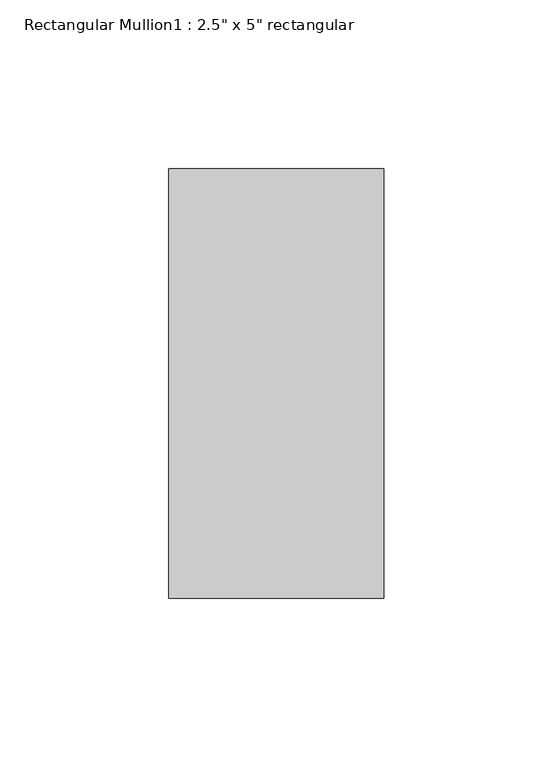
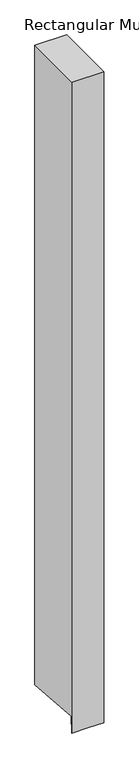
"""IFC4 building model written with IfcOpenShell, lengths in millimetres: member geometry."""

import ifcopenshell
import ifcopenshell.guid

model = None  # the IFC model being written
_history = None  # IfcOwnerHistory: only IFC2X3 demands one
_inside = {}  # id of a spatial element -> (the spatial element, [elements in it])
_under = {}  # id of a project, library or spatial element -> (it, [spatial elements below it])
_declared = {}  # id of a project -> (the project, [libraries it declares])
_typed = {}  # id of a type object -> (the type object, [elements of that type])
_made_of = {}  # id of a material, layer set ... -> (it, [elements and type objects made of it])


def new_model(schema):
    """Start an empty IFC model of exactly this schema.

    Asked for "IFC4X3", IfcOpenShell would pick the latest addendum, in which some entities
    have other attributes; the version numbers below select the first issue.
    IFC2X3 requires an IfcOwnerHistory on every rooted entity: one is made here for all.
    """
    global model, _history
    if schema == "IFC4X3":
        model = ifcopenshell.file(schema_version=(4, 3, 0, 0))
    else:
        model = ifcopenshell.file(schema=schema)
    _inside.clear()
    _under.clear()
    _declared.clear()
    _typed.clear()
    _made_of.clear()
    _history = None
    if model.schema == "IFC2X3":
        org = make("IfcOrganization", Name="unknown")
        user = make(
            "IfcPersonAndOrganization",
            ThePerson=make("IfcPerson", FamilyName="unknown"),
            TheOrganization=org,
        )
        app = make(
            "IfcApplication",
            ApplicationDeveloper=org,
            Version="unknown",
            ApplicationFullName="unknown",
            ApplicationIdentifier="unknown",
        )
        _history = make(
            "IfcOwnerHistory",
            OwningUser=user,
            OwningApplication=app,
            ChangeAction="ADDED",
            CreationDate=0,
        )
    return model


def make(cls, **values):
    """One entity of the class cls with the attributes given. An attribute that is None is left unset."""
    return model.create_entity(
        cls, **{name: value for name, value in values.items() if value is not None}
    )


def rooted(cls, **values):
    """An entity with a GlobalId (a new one), such as an element, a storey or a relation."""
    return make(cls, GlobalId=ifcopenshell.guid.new(), OwnerHistory=_history, **values)


def si_unit(unit_type, name, prefix=None):
    """IfcSIUnit, for example si_unit("LENGTHUNIT", "METRE", prefix="MILLI")."""
    return make("IfcSIUnit", UnitType=unit_type, Prefix=prefix, Name=name)


def assignment(units):
    """IfcUnitAssignment: the units of a project."""
    return None if units is None else make("IfcUnitAssignment", Units=units)


def point(xyz):
    """IfcCartesianPoint."""
    return None if xyz is None else make("IfcCartesianPoint", Coordinates=xyz)


def direction(xyz):
    """IfcDirection."""
    return None if xyz is None else make("IfcDirection", DirectionRatios=xyz)


def frame(location, z_axis=None, x_axis=None):
    """IfcAxis2Placement3D, a coordinate frame: its origin and axes. An axis left out is left unset."""
    return make(
        "IfcAxis2Placement3D",
        Location=point(location),
        Axis=direction(z_axis),
        RefDirection=direction(x_axis),
    )


def origin():
    """The frame at (0, 0, 0) with its axes left unset."""
    return frame((0.0, 0.0, 0.0))


def place(relative_to, where):
    """IfcLocalPlacement: puts the frame where relative to a parent placement (None: the world)."""
    return make(
        "IfcLocalPlacement", PlacementRelTo=relative_to, RelativePlacement=where
    )


def context(
    kind, dimensions, precision=None, world=None, true_north=None, identifier=None
):
    """IfcGeometricRepresentationContext, for example the 3D "Model" context."""
    return make(
        "IfcGeometricRepresentationContext",
        ContextIdentifier=identifier,
        ContextType=kind,
        CoordinateSpaceDimension=dimensions,
        Precision=precision,
        WorldCoordinateSystem=world,
        TrueNorth=true_north,
    )


def project(units=None, contexts=None):
    """IfcProject with its units and contexts."""
    return rooted(
        "IfcProject",
        Name="project",
        RepresentationContexts=contexts,
        UnitsInContext=assignment(units),
    )


def spatial(cls, under=None, at=None, **own):
    """A site, building, storey or space (cls), placed at a placement, below another one or the project."""
    s = rooted(cls, ObjectPlacement=at, **own)
    if under is not None:
        _under.setdefault(under.id(), (under, []))[1].append(s)
    return s


def faces_of(points, faces, orient=None, outer=None):
    """IfcFace entities. A face is a list of loops; a loop is a list of indices into points, from 0.

    orient and outer hold one flag for each loop. By default every Orientation is true, the
    first loop of a face is its IfcFaceOuterBound and the others are IfcFaceBound.
    """
    made = []
    for i, loops in enumerate(faces):
        bounds = []
        for j, loop in enumerate(loops):
            is_outer = j == 0 if outer is None else outer[i][j]
            bounds.append(
                make(
                    "IfcFaceOuterBound" if is_outer else "IfcFaceBound",
                    Bound=make("IfcPolyLoop", Polygon=[points[k] for k in loop]),
                    Orientation=True if orient is None else orient[i][j],
                )
            )
        made.append(make("IfcFace", Bounds=bounds))
    return made


def faceted_brep(points, faces, orient=None, outer=None, voids=None):
    """IfcFacetedBrep: a solid bounded by flat faces; with voids (closed shells), ...WithVoids."""
    shared = [point(p) for p in points]
    hull = make("IfcClosedShell", CfsFaces=faces_of(shared, faces, orient, outer))
    if voids is None:
        return make("IfcFacetedBrep", Outer=hull)
    return make(
        "IfcFacetedBrepWithVoids",
        Outer=hull,
        Voids=[
            make(cls, CfsFaces=faces_of(shared, fs, o, b)) for cls, fs, o, b in voids
        ],
    )


def shape(context_of_items, identifier, shape_type, items):
    """IfcShapeRepresentation: the items that make up one representation, for example the "Body"."""
    return make(
        "IfcShapeRepresentation",
        ContextOfItems=context_of_items,
        RepresentationIdentifier=identifier,
        RepresentationType=shape_type,
        Items=items,
    )


def source(mapping_origin, context_of_items, identifier, shape_type, items):
    """IfcRepresentationMap: a shape defined once, which mapped items show again and again."""
    return make(
        "IfcRepresentationMap",
        MappingOrigin=mapping_origin,
        MappedRepresentation=shape(context_of_items, identifier, shape_type, items),
    )


def transform(
    local_origin,
    x_axis=None,
    y_axis=None,
    z_axis=None,
    scale=None,
    scale2=None,
    scale3=None,
    uniform=True,
):
    """IfcCartesianTransformationOperator3D, or its non-uniform kind. x_axis, y_axis, z_axis: its Axis1, 2, 3."""
    if uniform:
        return make(
            "IfcCartesianTransformationOperator3D",
            Axis1=direction(x_axis),
            Axis2=direction(y_axis),
            LocalOrigin=point(local_origin),
            Scale=scale,
            Axis3=direction(z_axis),
        )
    return make(
        "IfcCartesianTransformationOperator3DnonUniform",
        Axis1=direction(x_axis),
        Axis2=direction(y_axis),
        LocalOrigin=point(local_origin),
        Scale=scale,
        Axis3=direction(z_axis),
        Scale2=scale2,
        Scale3=scale3,
    )


def mapped(mapping_source, mapping_target):
    """IfcMappedItem: shows the shape of a source again, moved by a transform."""
    return make(
        "IfcMappedItem", MappingSource=mapping_source, MappingTarget=mapping_target
    )


def made_of(thing, what):
    """Note that an element or type object is made of a material, layer set ...; save() writes the relation."""
    if what is not None:
        _made_of.setdefault(what.id(), (what, []))[1].append(thing)
    return thing


def element(
    cls,
    number,
    at=None,
    inside=None,
    cuts=None,
    type_object=None,
    material=None,
    context=None,
    identifier="Body",
    shape_type=None,
    held_by="IfcProductDefinitionShape",
    body=None,
    shapes=None,
    **own,
):
    """One element of the class cls, such as IfcWall. Its Tag is "e" and its number.

    at: its placement. inside: the storey or other place that contains it. cuts: it is an
    opening in that element (IfcRelVoidsElement). A single representation is given by context,
    identifier, shape_type and body (its items); several are given by shapes. held_by: the class
    of the entity that holds the representations. save() writes the other relations.
    """
    e = rooted(cls, Tag="e%d" % number, ObjectPlacement=at, **own)
    if body is not None:
        shapes = [shape(context, identifier, shape_type, body)]
    if shapes is not None:
        e.Representation = make(held_by, Representations=shapes)
    if inside is not None:
        _inside.setdefault(inside.id(), (inside, []))[1].append(e)
    if cuts is not None:
        rooted(
            "IfcRelVoidsElement", RelatingBuildingElement=cuts, RelatedOpeningElement=e
        )
    if type_object is not None:
        _typed.setdefault(type_object.id(), (type_object, []))[1].append(e)
    return made_of(e, material)


def aggregate(whole, parts):
    """IfcRelAggregates: a whole, such as a stair, and the parts it consists of."""
    return rooted("IfcRelAggregates", RelatingObject=whole, RelatedObjects=parts)


def save(model, path):
    """Write the relations noted so far, then the file.

    IfcRelAggregates (storeys below a building ...), IfcRelContainedInSpatialStructure (elements
    in a storey), IfcRelDefinesByType, IfcRelAssociatesMaterial and IfcRelDeclares: one each for
    every whole, place, type object, material and project.
    """
    for whole, parts in _under.values():
        aggregate(whole, parts)
    for where, things in _inside.values():
        rooted(
            "IfcRelContainedInSpatialStructure",
            RelatedElements=things,
            RelatingStructure=where,
        )
    for kind, things in _typed.values():
        rooted("IfcRelDefinesByType", RelatedObjects=things, RelatingType=kind)
    for what, things in _made_of.values():
        rooted("IfcRelAssociatesMaterial", RelatedObjects=things, RelatingMaterial=what)
    for by, libraries in _declared.values():
        rooted("IfcRelDeclares", RelatingContext=by, RelatedDefinitions=libraries)
    model.write(path)


def member_275a0903(model_context):
    return source(origin(), model_context, "Body", "Brep", [
        faceted_brep([(31.75, 63.5, 0.0), (-31.75, 63.5, 0.0), (-31.75, -63.5, 0.0), (31.75, -63.5, 0.0), (31.75, 63.5, -1344.0500431), (0.0, 63.5, -1344.0500431), (-31.75, 63.5, -1344.0500431), (-31.75, -60.9736199, -1334.8041085), (-31.75, -63.5, -1368.815562), (0.0, -63.5, -1368.815562), (31.75, -63.5, -1368.815562), (31.75, -60.9736199, -1334.8041085), (0.0, -60.9736199, -1334.8041085)], [[[0, 1, 2, 3]], [[1, 0, 4, 5, 6]], [[2, 1, 6, 7, 8]], [[3, 2, 8, 9, 10]], [[0, 3, 10, 11, 4]], [[4, 11, 12, 5]], [[11, 10, 9, 12]], [[9, 8, 7, 12]], [[7, 6, 5, 12]]]),
    ])


if __name__ == "__main__":
    model = new_model("IFC4")
    model_context = context("Model", 3, world=origin())
    ifc_project = project(units=[si_unit("LENGTHUNIT", "METRE", prefix="MILLI")], contexts=[model_context])
    site = spatial("IfcSite", under=ifc_project)
    building = spatial("IfcBuilding", under=site)
    placement = place(None, origin())
    member_shape = member_275a0903(model_context)
    element("IfcMember", 1, ObjectType="Rectangular Mullion1 : 2.5\" x 5\" rectangular", at=placement, inside=building, context=model_context, shape_type="MappedRepresentation", body=[
        mapped(member_shape, transform((0.0, 0.0, 0.0), x_axis=(1.0, 0.0, 0.0), y_axis=(0.0, 1.0, 0.0), z_axis=(0.0, 0.0, 1.0))),
    ])
    save(model, "model.ifc")

# Revit data of these elements
# Type "Rectangular Mullion1 : 2.5\" x 5\" rectangular"
#   built-in parameter 1007304 = 0.416667 (stored number, unit not read)
#   built-in parameter 1007301 = 0.104167 (stored number, unit not read)
#   built-in parameter 1007300 = 0.104167 (stored number, unit not read)
# Element 1 (IfcMember, "Rectangular Mullion1 : 2.5\" x 5\" rectangular")
#   Materials on its faces: "support-frame"
# Materials
#   "support-frame": class "Unassigned", colour RGB 233 233 233, transparency 0, Cost = 0
